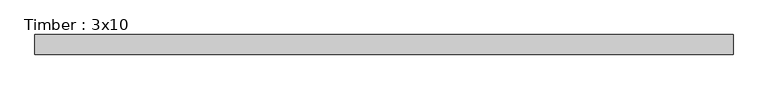
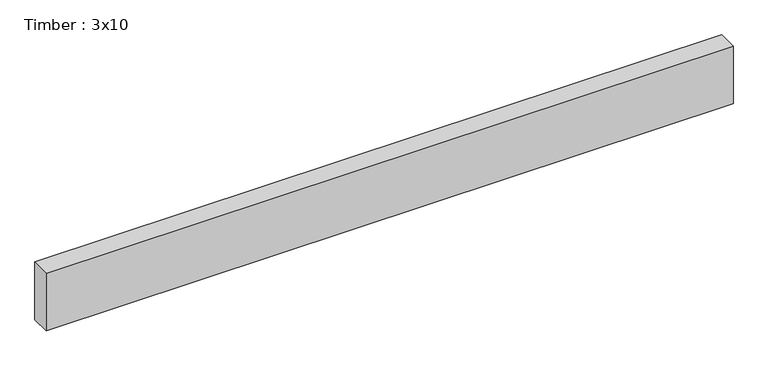
"""IFC4 building model written with IfcOpenShell, lengths in millimetres: beam geometry, Timber : 3x10."""

from ifc_helpers import new_model, si_unit, frame, origin, place, context, project, spatial, polyline, outline, extrude, source, transform, mapped, element, save


def timber_3x10_5e682144(model_context):
    return source(origin(), model_context, "Body", "SweptSolid", [
        extrude(outline(polyline([(1352.55, 38.1), (1352.55, -38.1), (-1352.55, -38.1), (-1352.55, 38.1), (1352.55, 38.1)])), frame((0.0, 0.0, -120.65), z_axis=(0.0, 0.0, 1.0), x_axis=(1.0, 0.0, 0.0)), (0.0, 0.0, 1.0), 241.3),
    ])


if __name__ == "__main__":
    model = new_model("IFC4")
    model_context = context("Model", 3, world=origin())
    ifc_project = project(units=[si_unit("LENGTHUNIT", "METRE", prefix="MILLI")], contexts=[model_context])
    site = spatial("IfcSite", under=ifc_project)
    building = spatial("IfcBuilding", under=site)
    placement = place(None, origin())
    timber_3x10_shape = timber_3x10_5e682144(model_context)
    element("IfcBeam", 1, ObjectType="Timber : 3x10", at=placement, inside=building, context=model_context, shape_type="MappedRepresentation", body=[
        mapped(timber_3x10_shape, transform((0.0, 0.0, 0.0), x_axis=(1.0, 0.0, 0.0), y_axis=(0.0, 1.0, 0.0), z_axis=(0.0, 0.0, 1.0))),
    ])
    save(model, "model.ifc")

# Revit data of these elements
# Type "Timber : 3x10"
#   Assembly Code = "B10"
#   A = 0.362847 SF
#   Length [instance default] = 5' - 0"
#   b = 0' - 3"
#   d = 0' - 9 1/2"
#   Structural Material [instance default] = Softwood, Lumber
# Element 1 (IfcBeam, "Timber : 3x10")
#   Materials on its faces: "Softwood, Lumber"
# Materials
#   "Softwood, Lumber": class "Wood", colour RGB 144 113 62, transparency 0, Description = "Pinus Echinata", Cost = 0
